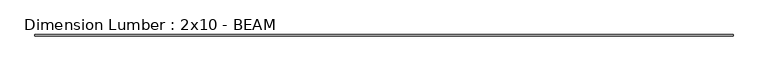
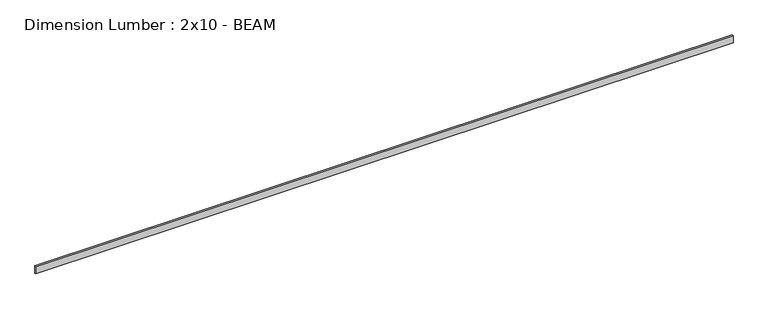
"""IFC4 building model written with IfcOpenShell, lengths in millimetres: beam geometry, Dimension Lumber : 2x10 - BEAM."""

from ifc_helpers import new_model, si_unit, frame, origin, place, context, project, spatial, polyline, outline, extrude, source, transform, mapped, element, save


def dimension_lumber_2x10_beam_1127f659(model_context):
    return source(origin(), model_context, "Body", "SweptSolid", [
        extrude(outline(polyline([(10604.4219826, 19.05), (10604.4219826, -19.05), (-10798.4018456, -19.05), (-10798.4018456, 19.05), (10604.4219826, 19.05)])), frame((0.0, 0.0, -117.475), z_axis=(0.0, 0.0, 1.0), x_axis=(1.0, 0.0, 0.0)), (0.0, 0.0, 1.0), 234.95),
    ])


if __name__ == "__main__":
    model = new_model("IFC4")
    model_context = context("Model", 3, world=origin())
    ifc_project = project(units=[si_unit("LENGTHUNIT", "METRE", prefix="MILLI")], contexts=[model_context])
    site = spatial("IfcSite", under=ifc_project)
    building = spatial("IfcBuilding", under=site)
    placement = place(None, origin())
    dimension_lumber_2x10_beam_shape = dimension_lumber_2x10_beam_1127f659(model_context)
    element("IfcBeam", 1, ObjectType="Dimension Lumber : 2x10 - BEAM", at=placement, inside=building, context=model_context, shape_type="MappedRepresentation", body=[
        mapped(dimension_lumber_2x10_beam_shape, transform((0.0, 0.0, 0.0), x_axis=(1.0, 0.0, 0.0), y_axis=(0.0, 1.0, 0.0), z_axis=(0.0, 0.0, 1.0))),
    ])
    save(model, "model.ifc")

# Revit data of these elements
# Type "Dimension Lumber : 2x10 - BEAM"
#   Assembly Code = "B10"
#   A = 0.0755556 SF
#   Length [instance default] = 5' - 0"
#   b = 0' - 1 1/2"
#   d = 0' - 9 1/4"
#   Structural Material = (3) SISTERED 2X10s AT BEAM
# Element 1 (IfcBeam, "Dimension Lumber : 2x10 - BEAM")
#   Materials on its faces: "(3) SISTERED 2X10s AT BEAM"
# Materials
#   "(3) SISTERED 2X10s AT BEAM": class "Wood", colour RGB 234 198 147, transparency 0, Description = "Pinus Echinata", Cost = 0
